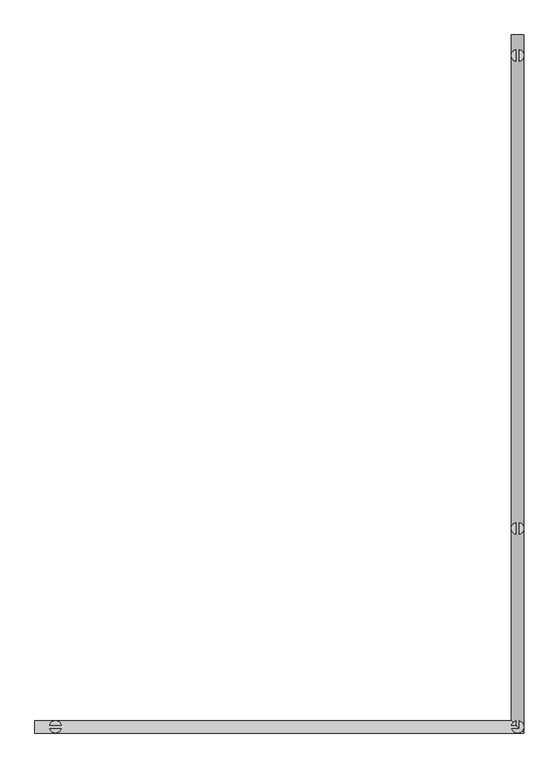
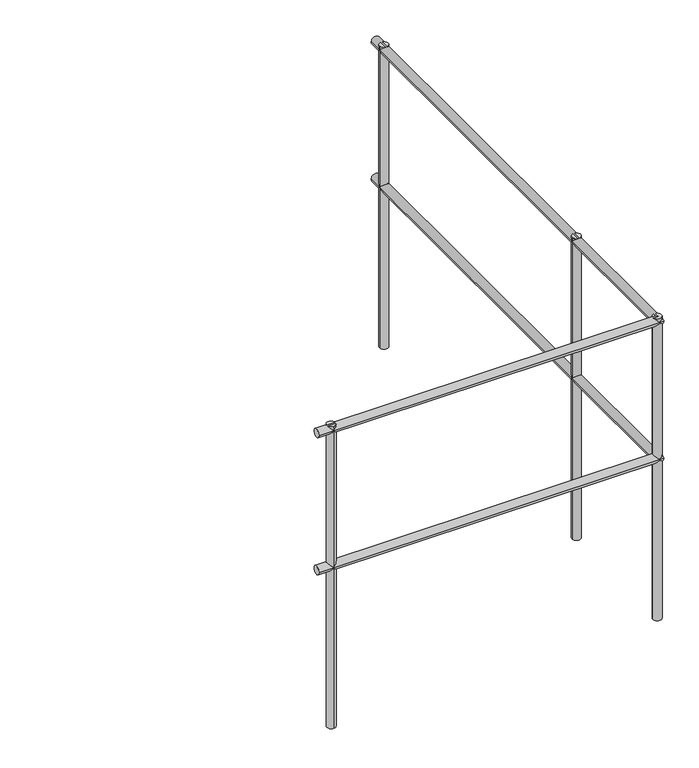
"""IFC4 building model written with IfcOpenShell, lengths in millimetres: railing geometry."""

from ifc_helpers import new_model, si_unit, point, frame, frame_2d, origin, place, context, project, spatial, circle_curve, ellipse_curve, trimmed, segment, composite_curve, outline, extrude, source, transform, mapped, element, save
from ifc_brep_helpers import plane_surface, cylinder_surface, advanced_brep


def railing_da86e9fc(model_context):
    return source(origin(), model_context, "Body", "SolidModel", [
        advanced_brep(
        [(11414.7052251, 14979.5208589, 4745.0), (11384.7052251, 14979.5208589, 4745.0), (10225.0, 13282.0208589, 4745.0), (10225.0, 13312.0208589, 4745.0), (11414.7052251, 13282.0208589, 4745.0), (11384.7052251, 13312.0208589, 4745.0)],
        [
            (0, 1, circle_curve(frame((11399.7052251, 14979.5208589, 4745.0), z_axis=(0.0, 1.0, 0.0), x_axis=(-1.0, 0.0, 0.0)), 15.0)),
            (1, 0, circle_curve(frame((11399.7052251, 14979.5208589, 4745.0), z_axis=(0.0, 1.0, 0.0), x_axis=(-1.0, 0.0, 0.0)), 15.0)),
            (2, 3, circle_curve(frame((10225.0, 13297.0208589, 4745.0), z_axis=(-1.0, 0.0, 0.0), x_axis=(0.0, 1.0, 0.0)), 15.0)),
            (3, 2, circle_curve(frame((10225.0, 13297.0208589, 4745.0), z_axis=(-1.0, 0.0, 0.0), x_axis=(0.0, 1.0, 0.0)), 15.0)),
            (0, 4),
            (4, 5, ellipse_curve(frame((11399.7052251, 13297.0208589, 4745.0), z_axis=(0.7071067811865493, 0.7071067811865457, 0.0), x_axis=(-0.7071067811865457, 0.7071067811865493, 0.0)), 21.2132034, 15.0)),
            (5, 1),
            (5, 4, ellipse_curve(frame((11399.7052251, 13297.0208589, 4745.0), z_axis=(0.7071067811865493, 0.7071067811865457, 0.0), x_axis=(-0.7071067811865457, 0.7071067811865493, 0.0)), 21.2132034, 15.0)),
            (4, 2),
            (3, 5),
        ],
        [
            plane_surface(frame((11399.7052251, 14979.5208589, 4760.0), z_axis=(0.0, 1.0, 0.0), x_axis=(0.0, 0.0, -1.0))),
            plane_surface(frame((10225.0, 13297.0208589, 4760.0), z_axis=(-1.0, 0.0, 0.0), x_axis=(0.0, -1.0, 0.0))),
            cylinder_surface(frame((11399.7052251, 14979.5208589, 4745.0), z_axis=(0.0, 1.0, 0.0), x_axis=(-1.0, 0.0, 0.0)), 15.0),
            cylinder_surface(frame((11399.7052251, 13297.0208589, 4745.0), z_axis=(1.0, 0.0, 0.0), x_axis=(0.0, 1.0, 0.0)), 15.0),
        ],
        [
            (0, [[1, 2]]),
            (1, [[3, 4]]),
            (2, [[-1, 5, 6, 7]]),
            (2, [[-2, -7, 8, -5]]),
            (3, [[-6, 9, -4, 10]]),
            (3, [[-8, -10, -3, -9]]),
        ],
    ),
        advanced_brep(
        [(11414.7052251, 14979.5208589, 5245.0), (11384.7052251, 14979.5208589, 5245.0), (11414.7052251, 13282.0208589, 5245.0), (11384.7052251, 13312.0208589, 5245.0), (10225.0, 13282.0208589, 5245.0), (10225.0, 13312.0208589, 5245.0)],
        [
            (0, 1, circle_curve(frame((11399.7052251, 14979.5208589, 5245.0), z_axis=(0.0, 1.0, 0.0), x_axis=(-1.0, 0.0, 0.0)), 15.0)),
            (1, 0, circle_curve(frame((11399.7052251, 14979.5208589, 5245.0), z_axis=(0.0, 1.0, 0.0), x_axis=(-1.0, 0.0, 0.0)), 15.0)),
            (0, 2),
            (2, 3, ellipse_curve(frame((11399.7052251, 13297.0208589, 5245.0), z_axis=(0.7071067811865493, 0.7071067811865457, 0.0), x_axis=(-0.7071067811865457, 0.7071067811865493, 0.0)), 21.2132034, 15.0)),
            (3, 1),
            (3, 2, ellipse_curve(frame((11399.7052251, 13297.0208589, 5245.0), z_axis=(0.7071067811865493, 0.7071067811865457, 0.0), x_axis=(-0.7071067811865457, 0.7071067811865493, 0.0)), 21.2132034, 15.0)),
            (4, 5, circle_curve(frame((10225.0, 13297.0208589, 5245.0), z_axis=(-1.0, 0.0, 0.0), x_axis=(0.0, 1.0, 0.0)), 15.0)),
            (5, 4, circle_curve(frame((10225.0, 13297.0208589, 5245.0), z_axis=(-1.0, 0.0, 0.0), x_axis=(0.0, 1.0, 0.0)), 15.0)),
            (2, 4),
            (5, 3),
        ],
        [
            plane_surface(frame((11399.7052251, 14979.5208589, 5260.0), z_axis=(0.0, 1.0, 0.0), x_axis=(0.0, 0.0, -1.0))),
            cylinder_surface(frame((11399.7052251, 14979.5208589, 5245.0), z_axis=(0.0, 1.0, 0.0), x_axis=(-1.0, 0.0, 0.0)), 15.0),
            plane_surface(frame((10225.0, 13297.0208589, 5260.0), z_axis=(-1.0, 0.0, 0.0), x_axis=(0.0, -1.0, 0.0))),
            cylinder_surface(frame((11399.7052251, 13297.0208589, 5245.0), z_axis=(1.0, 0.0, 0.0), x_axis=(0.0, 1.0, 0.0)), 15.0),
        ],
        [
            (0, [[1, 2]]),
            (1, [[-1, 3, 4, 5]]),
            (1, [[-2, -5, 6, -3]]),
            (2, [[7, 8]]),
            (3, [[-4, 9, -8, 10]]),
            (3, [[-6, -10, -7, -9]]),
        ],
    ),
        extrude(outline(composite_curve([segment(trimmed(circle_curve(frame_2d((11399.7052251, 13779.5208589)), 15.0), [point((11384.7052251, 13779.5208589))], [point((11414.7052251, 13779.5208589))], False, "CARTESIAN"), True, "CONTINUOUS"), segment(trimmed(circle_curve(frame_2d((11399.7052251, 13779.5208589)), 15.0), [point((11414.7052251, 13779.5208589))], [point((11384.7052251, 13779.5208589))], False, "CARTESIAN"), True, "CONTINUOUS")], self_intersect=False)), frame((0.0, 0.0, 4160.0), z_axis=(0.0, 0.0, 1.0), x_axis=(1.0, 0.0, 0.0)), (0.0, 0.0, 1.0), 1100.0),
        extrude(outline(composite_curve([segment(trimmed(circle_curve(frame_2d((11399.7052251, 13297.0208589)), 15.0), [point((11384.7052251, 13297.0208589))], [point((11414.7052251, 13297.0208589))], False, "CARTESIAN"), True, "CONTINUOUS"), segment(trimmed(circle_curve(frame_2d((11399.7052251, 13297.0208589)), 15.0), [point((11414.7052251, 13297.0208589))], [point((11384.7052251, 13297.0208589))], False, "CARTESIAN"), True, "CONTINUOUS")], self_intersect=False)), frame((0.0, 0.0, 4160.0), z_axis=(0.0, 0.0, 1.0), x_axis=(1.0, 0.0, 0.0)), (0.0, 0.0, 1.0), 1100.0),
        extrude(outline(composite_curve([segment(trimmed(circle_curve(frame_2d((10275.0, 13297.0208589)), 15.0), [point((10275.0, 13312.0208589))], [point((10275.0, 13282.0208589))], False, "CARTESIAN"), True, "CONTINUOUS"), segment(trimmed(circle_curve(frame_2d((10275.0, 13297.0208589)), 15.0), [point((10275.0, 13282.0208589))], [point((10275.0, 13312.0208589))], False, "CARTESIAN"), True, "CONTINUOUS")], self_intersect=False)), frame((0.0, 0.0, 4160.0), z_axis=(0.0, 0.0, 1.0), x_axis=(1.0, 0.0, 0.0)), (0.0, 0.0, 1.0), 1100.0),
        extrude(outline(composite_curve([segment(trimmed(circle_curve(frame_2d((11399.7052251, 14929.5208589)), 15.0), [point((11384.7052251, 14929.5208589))], [point((11414.7052251, 14929.5208589))], False, "CARTESIAN"), True, "CONTINUOUS"), segment(trimmed(circle_curve(frame_2d((11399.7052251, 14929.5208589)), 15.0), [point((11414.7052251, 14929.5208589))], [point((11384.7052251, 14929.5208589))], False, "CARTESIAN"), True, "CONTINUOUS")], self_intersect=False)), frame((0.0, 0.0, 4160.0), z_axis=(0.0, 0.0, 1.0), x_axis=(1.0, 0.0, 0.0)), (0.0, 0.0, 1.0), 1100.0),
    ])


if __name__ == "__main__":
    model = new_model("IFC4")
    model_context = context("Model", 3, world=origin())
    ifc_project = project(units=[si_unit("LENGTHUNIT", "METRE", prefix="MILLI")], contexts=[model_context])
    site = spatial("IfcSite", under=ifc_project)
    building = spatial("IfcBuilding", under=site)
    placement = place(None, origin())
    railing_shape = railing_da86e9fc(model_context)
    element("IfcRailing", 1, at=placement, inside=building, context=model_context, shape_type="MappedRepresentation", body=[
        mapped(railing_shape, transform((0.0, 0.0, 0.0), x_axis=(1.0, 0.0, 0.0), y_axis=(0.0, 1.0, 0.0), z_axis=(0.0, 0.0, 1.0))),
    ])
    save(model, "model.ifc")
